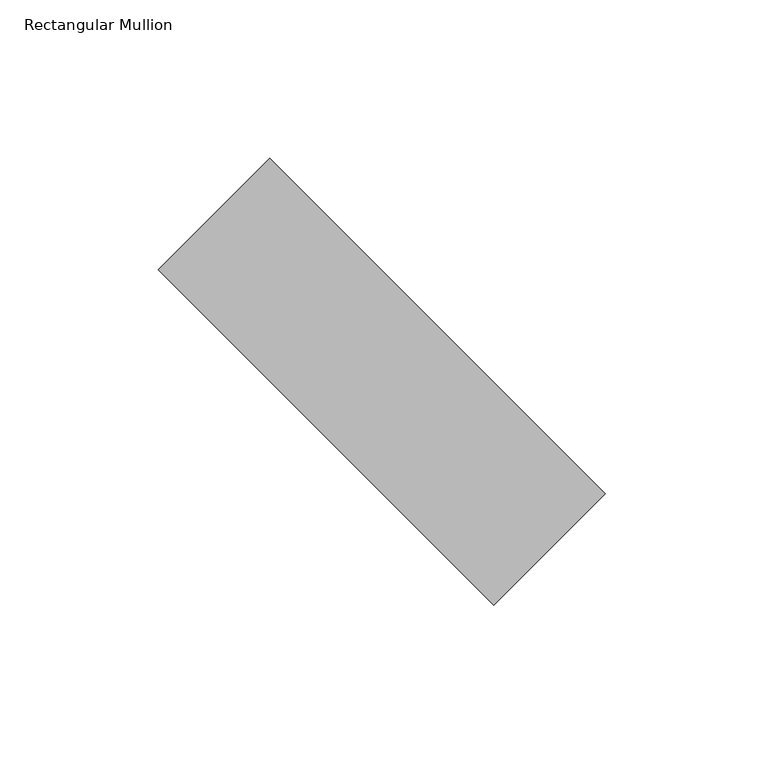
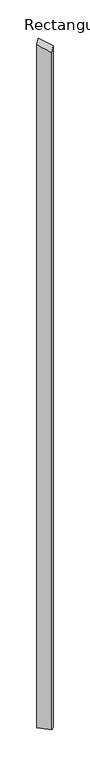
"""IFC4 building model written with IfcOpenShell, lengths in millimetres: member geometry, Rectangular Mullion : tilted mullions."""

from ifc_helpers import new_model, si_unit, origin, place, context, project, spatial, faceted_brep, source, transform, mapped, element, save


def rectangular_mullion_25b424f6(model_context):
    return source(origin(), model_context, "Body", "Brep", [
        faceted_brep([(-35.3553391, 70.7106781, -7999.9632991), (70.7106781, -35.3553391, -7999.9632991), (35.3553391, -70.7106781, -7999.9632991), (-70.7106781, 35.3553391, -7999.9632991), (-70.7106781, 35.3553391, 9.9623104), (-35.3553391, 70.7106781, 55.0258879), (35.3553391, -70.7106781, -55.0258879), (70.7106781, -35.3553391, -9.9623104)], [[[0, 1, 2, 3]], [[4, 5, 0, 3]], [[6, 4, 3, 2]], [[7, 6, 2, 1]], [[5, 7, 1, 0]], [[5, 4, 6, 7]]]),
    ])


if __name__ == "__main__":
    model = new_model("IFC4")
    model_context = context("Model", 3, world=origin())
    ifc_project = project(units=[si_unit("LENGTHUNIT", "METRE", prefix="MILLI")], contexts=[model_context])
    site = spatial("IfcSite", under=ifc_project)
    building = spatial("IfcBuilding", under=site)
    placement = place(None, origin())
    rectangular_mullion_shape = rectangular_mullion_25b424f6(model_context)
    element("IfcMember", 1, ObjectType="Rectangular Mullion : tilted mullions", at=placement, inside=building, context=model_context, shape_type="MappedRepresentation", body=[
        mapped(rectangular_mullion_shape, transform((0.0, 0.0, 0.0), x_axis=(1.0, 0.0, 0.0), y_axis=(0.0, 1.0, 0.0), z_axis=(0.0, 0.0, 1.0))),
    ])
    save(model, "model.ifc")

# Revit data of these elements
# Type "Rectangular Mullion : tilted mullions"
#   built-in parameter 1007304 = 0.492126 (stored number, unit not read)
#   built-in parameter 1007301 = 0.082021 (stored number, unit not read)
#   built-in parameter 1007300 = 0.082021 (stored number, unit not read)
# Element 1 (IfcMember, "Rectangular Mullion : tilted mullions")
#   Materials on its faces: "Aluminum"
# Materials
#   "Aluminum": class "Metal", colour RGB 244 244 244, transparency 0, Description = "Aluminum 6061", Cost = 0
